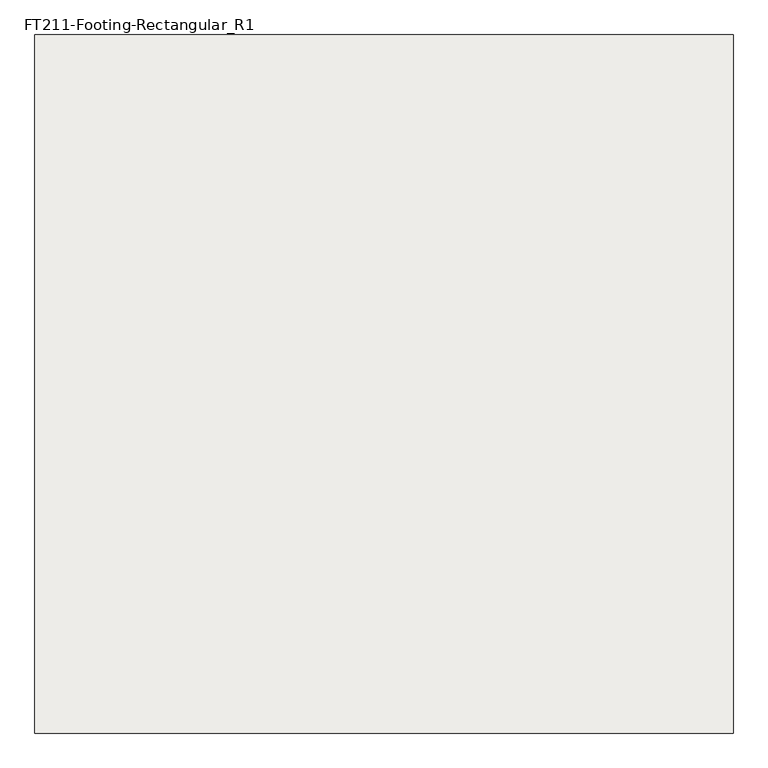
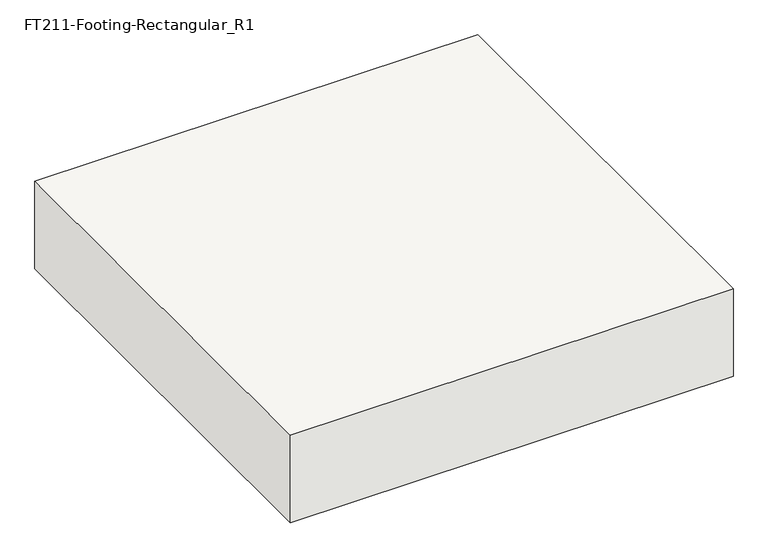
"""IFC4 building model written with IfcOpenShell, lengths in millimetres: slab geometry, FT211-Footing-Rectangular_R1 : H_SF_ACF_W2400xL2400xT500_Bitumen."""

from ifc_helpers import new_model, si_unit, frame, origin, place, context, project, spatial, polyline, outline, extrude, source, transform, mapped, element, save


def ft211_footing_rectangular_r1_5fe39465(model_context):
    return source(origin(), model_context, "Body", "SweptSolid", [
        extrude(outline(polyline([(1200.0, 1200.0), (1200.0, -1200.0), (-1200.0, -1200.0), (-1200.0, 1200.0), (1200.0, 1200.0)])), frame((0.0, 0.0, -500.0), z_axis=(0.0, 0.0, 1.0), x_axis=(1.0, 0.0, 0.0)), (0.0, 0.0, 1.0), 500.0),
    ])


if __name__ == "__main__":
    model = new_model("IFC4")
    model_context = context("Model", 3, world=origin())
    ifc_project = project(units=[si_unit("LENGTHUNIT", "METRE", prefix="MILLI")], contexts=[model_context])
    site = spatial("IfcSite", under=ifc_project)
    building = spatial("IfcBuilding", under=site)
    placement = place(None, origin())
    ft211_footing_rectangular_r1_shape = ft211_footing_rectangular_r1_5fe39465(model_context)
    element("IfcSlab", 1, ObjectType="FT211-Footing-Rectangular_R1 : H_SF_ACF_W2400xL2400xT500_Bitumen", at=placement, inside=building, context=model_context, shape_type="MappedRepresentation", body=[
        mapped(ft211_footing_rectangular_r1_shape, transform((0.0, 0.0, 0.0), x_axis=(1.0, 0.0, 0.0), y_axis=(0.0, 1.0, 0.0), z_axis=(0.0, 0.0, 1.0))),
    ])
    save(model, "model.ifc")

# Revit data of these elements
# Type "FT211-Footing-Rectangular_R1 : H_SF_ACF_W2400xL2400xT500_Bitumen"
#   Top bar = "D25@300"
#   Description = "UG Shallow Foundation"
#   Bottom bar = "D20@300"
#   Width = 2400 mm
#   Length = 2400 mm
#   Foundation Thickness = 500 mm
#   Structural Material [instance default] = none
#   Assembly Code = ""
